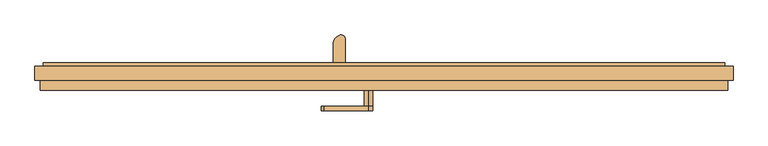
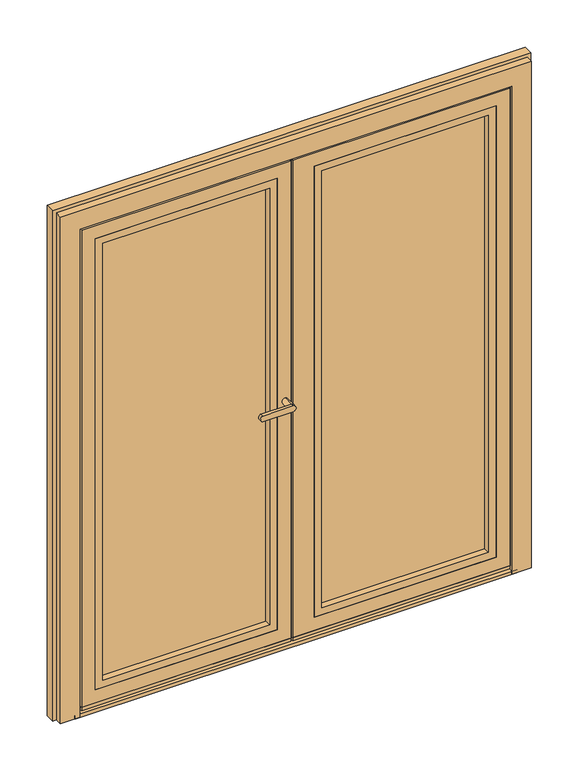
"""IFC4 building model written with IfcOpenShell, lengths in millimetres: door geometry, Schueco_FWS_ADS-75-BL-SimplySmart_out_Family-02 : FWS SI insert unit."""

from ifc_helpers import new_model, si_unit, point, frame, frame_2d, origin, place, context, project, spatial, polyline, circle_curve, ellipse_curve, trimmed, segment, composite_curve, outline, extrude, faceted_brep, source, transform, mapped, element, save
from ifc_brep_helpers import plane_surface, cylinder_surface, extruded_surface, advanced_brep


def door_16c4306f(model_context):
    return source(origin(), model_context, "Body", "SolidModel", [
        faceted_brep([(855.0, -57.5000065, 40.0), (855.0, -57.5000065, 2055.0), (855.0, -66.0002823, 2055.0), (855.0, -66.0002823, 40.0), (-12.5, -66.0002823, 40.0), (-12.5, -57.5000065, 40.0), (8.5, -57.5000065, 40.0), (865.0, -57.5000065, 30.0), (865.0, -57.5000065, 2065.0), (8.5, -57.5000065, 2065.0), (8.5, -57.5000065, 2055.0), (8.5, -57.5000065, 30.0), (-12.5, -66.0002823, 2055.0), (73.5, -66.0002823, 95.0), (73.5, -66.0002823, 2000.0), (800.0, -66.0002823, 2000.0), (800.0, -66.0002823, 95.0), (800.0, -2.0002726, 2000.0), (800.0, -2.0002726, 95.0), (73.5, -2.0002726, 95.0), (73.5, -2.0002726, 2000.0), (105.5, -2.0002726, 127.0), (105.5, -2.0002726, 1968.0), (768.0, -2.0002726, 1968.0), (768.0, -2.0002726, 127.0), (768.0, 8.9997177, 1968.0), (768.0, 8.9997177, 127.0), (105.5, 8.9997177, 127.0), (105.5, 8.9997177, 1968.0), (887.0, 8.9997177, 8.0), (19.5, 8.9997177, 8.0), (19.5, 8.9997177, 2087.0), (887.0, 8.9997177, 2087.0), (887.0, 0.4997603, 2087.0), (887.0, 0.4997603, 8.0), (19.5, 0.4997603, 8.0), (19.5, 0.4997603, 2087.0), (19.5, 0.4997603, 2065.0), (865.0, 0.4997603, 2065.0), (865.0, 0.4997603, 30.0), (19.5, 0.4997603, 30.0), (8.5, 0.4997603, 30.0), (8.5, 0.4997603, 2065.0), (-12.5, -57.5000065, 2055.0)], [[[0, 1, 2, 3]], [[3, 4, 5, 6, 0]], [[7, 8, 9, 10, 1, 0, 6, 11]], [[2, 12, 4, 3], [13, 14, 15, 16]], [[16, 15, 17, 18]], [[18, 19, 13, 16]], [[19, 20, 14, 13]], [[18, 17, 20, 19], [21, 22, 23, 24]], [[24, 23, 25, 26]], [[26, 27, 21, 24]], [[27, 28, 22, 21]], [[29, 30, 31, 32], [26, 25, 28, 27]], [[29, 32, 33, 34]], [[34, 35, 30, 29]], [[33, 36, 37, 38, 39, 40, 35, 34]], [[39, 38, 8, 7]], [[7, 11, 41, 40, 39]], [[11, 6, 10, 9, 42, 41]], [[1, 10, 43, 12, 2]], [[20, 17, 15, 14]], [[28, 25, 23, 22]], [[32, 31, 36, 33]], [[9, 8, 38, 37, 42]], [[43, 10, 6, 5]], [[4, 12, 43, 5]], [[37, 36, 31, 30, 35, 40]], [[40, 41, 42, 37]]]),
        extrude(outline(polyline([(95.0, 73.5), (95.0, 800.0), (2000.0, 800.0), (2000.0, 73.5), (95.0, 73.5)]), holes=[polyline([(125.0, 770.0), (125.0, 103.5), (1970.0, 103.5), (1970.0, 770.0), (125.0, 770.0)])]), frame((0.0, -66.0002823, 0.0), z_axis=(0.0, 1.0, 0.0), x_axis=(0.0, 0.0, 1.0)), (0.0, 0.0, 1.0), 26.0000097),
        extrude(outline(polyline([(73.5, -40.0002726), (73.5, -2.0002726), (800.0, -2.0002726), (800.0, -40.0002726), (73.5, -40.0002726)])), frame((0.0, 0.0, 95.0), z_axis=(0.0, 0.0, 1.0), x_axis=(1.0, 0.0, 0.0)), (0.0, 0.0, 1.0), 1905.0),
        extrude(outline(polyline([(855.0, -66.0002823), (-12.5, -66.0002823), (-12.5, -57.5003249), (855.0, -57.5003249), (855.0, -66.0002823)])), frame((0.0, 0.0, 26.0), z_axis=(0.0, 0.0, 1.0), x_axis=(1.0, 0.0, 0.0)), (0.0, 0.0, 1.0), 14.0),
        extrude(outline(composite_curve([segment(polyline([(-139.1673236, 8.9997177), (-139.1673236, 59.1618682)]), True, "CONTINUOUS"), segment(trimmed(circle_curve(frame_2d((-111.9889059, 59.1618682)), 27.1784177), [point((-139.1673236, 59.1618682))], [point((-121.5260015, 84.6120194))], False, "CARTESIAN"), True, "CONTINUOUS"), segment(trimmed(circle_curve(frame_2d((-117.4485005, 73.7310321)), 11.6198924), [point((-121.5260015, 84.6120194))], [point((-105.8286081, 73.7310321))], False, "CARTESIAN"), True, "CONTINUOUS"), segment(polyline([(-105.8286081, 73.7310321), (-105.8286081, 8.9997177), (-139.1673236, 8.9997177)]), True, "CONTINUOUS")], self_intersect=False)), frame((0.0, 0.0, 2030.9340013), z_axis=(0.0, 0.0, 1.0), x_axis=(1.0, 0.0, 0.0)), (0.0, 0.0, 1.0), 4.0),
        extrude(outline(polyline([(-139.1673236, 12.9997177), (-105.8286081, 12.9997177), (-105.8286081, 8.9997177), (-139.1673236, 8.9997177), (-139.1673236, 12.9997177)])), frame((0.0, 0.0, 2000.9340013), z_axis=(0.0, 0.0, 1.0), x_axis=(1.0, 0.0, 0.0)), (0.0, 0.0, 1.0), 30.0),
        extrude(outline(polyline([(-139.1673236, 12.9997177), (-105.8286081, 12.9997177), (-105.8286081, 8.9997177), (-139.1673236, 8.9997177), (-139.1673236, 12.9997177)])), frame((0.0, 0.0, 56.9340013), z_axis=(0.0, 0.0, 1.0), x_axis=(1.0, 0.0, 0.0)), (0.0, 0.0, 1.0), 30.0),
        extrude(outline(composite_curve([segment(polyline([(-139.1673236, 8.9997177), (-139.1673236, 59.1618682)]), True, "CONTINUOUS"), segment(trimmed(circle_curve(frame_2d((-111.9889059, 59.1618682)), 27.1784177), [point((-139.1673236, 59.1618682))], [point((-121.5260015, 84.6120194))], False, "CARTESIAN"), True, "CONTINUOUS"), segment(trimmed(circle_curve(frame_2d((-117.4485005, 73.7310321)), 11.6198924), [point((-121.5260015, 84.6120194))], [point((-105.8286081, 73.7310321))], False, "CARTESIAN"), True, "CONTINUOUS"), segment(polyline([(-105.8286081, 73.7310321), (-105.8286081, 8.9997177), (-139.1673236, 8.9997177)]), True, "CONTINUOUS")], self_intersect=False)), frame((0.0, 0.0, 52.9340013), z_axis=(0.0, 0.0, 1.0), x_axis=(1.0, 0.0, 0.0)), (0.0, 0.0, 1.0), 4.0),
        advanced_brep(
        [(-109.782924, 57.5977179, 2030.9340013), (-135.217076, 72.2821425, 2030.9340013), (-109.782924, 57.5977179, 56.9340013), (-135.217076, 72.2821425, 56.9340013)],
        [
            (0, 1, ellipse_curve(frame((-122.5, 64.9399302, 2030.9340013), z_axis=(0.0, 0.0, 1.0000000000000002), x_axis=(0.5000002582658958, 0.866025254674503, 0.0)), 21.5840887, 14.6844171)),
            (1, 0, ellipse_curve(frame((-122.5, 64.9399302, 2030.9340013), z_axis=(0.0, 0.0, 1.0000000000000002), x_axis=(0.5000002582658958, 0.866025254674503, 0.0)), 21.5840887, 14.6844171)),
            (2, 3, ellipse_curve(frame((-122.5, 64.9399302, 56.9340013), z_axis=(0.0, 0.0, -1.0000000000000002), x_axis=(-0.866025254674503, 0.5000002582658958, 0.0)), 14.6844171, 21.5840887)),
            (3, 2, ellipse_curve(frame((-122.5, 64.9399302, 56.9340013), z_axis=(0.0, 0.0, -1.0000000000000002), x_axis=(-0.866025254674503, 0.5000002582658958, 0.0)), 14.6844171, 21.5840887)),
            (0, 2),
            (3, 1),
        ],
        [
            plane_surface(frame((-135.217076, 72.2821425, 2030.9340013), z_axis=(0.0, 0.0, 1.0000000000000002), x_axis=(0.5000002582658958, 0.866025254674503, 0.0))),
            plane_surface(frame((-135.217076, 72.2821425, 56.9340013), z_axis=(0.0, 0.0, -1.0000000000000002), x_axis=(-0.5000002582658958, -0.866025254674503, 0.0))),
            extruded_surface(trimmed(ellipse_curve(frame((-122.5, 64.9399302, 56.9340013), z_axis=(0.0, 0.0, -1.0000000000000002), x_axis=(-0.866025254674503, 0.5000002582658958, 0.0)), 14.6844171, 21.5840887), [point((-135.217076, 72.2821425, 56.9340013))], [point((-109.782924, 57.5977179, 56.9340013))], True, "CARTESIAN"), (0.0, 0.0, -1974.0), 1974.0),
            extruded_surface(trimmed(ellipse_curve(frame((-122.5, 64.9399302, 56.9340013), z_axis=(0.0, 0.0, -1.0000000000000002), x_axis=(-0.866025254674503, 0.5000002582658958, 0.0)), 14.6844171, 21.5840887), [point((-109.782924, 57.5977179, 56.9340013))], [point((-135.217076, 72.2821425, 56.9340013))], True, "CARTESIAN"), (0.0, 0.0, -1974.0), 1974.0),
        ],
        [
            (0, [[1, 2]]),
            (1, [[3, 4]]),
            (2, [[5, -4, 6, -1]]),
            (3, [[-6, -3, -5, -2]]),
        ],
    ),
        advanced_brep(
        [(-42.5, -122.0002518, 1038.0113692), (-42.5, -122.0002518, 1061.9886308), (-164.1617926, -122.0002518, 1061.9886308), (-164.1617926, -122.0002518, 1038.0113692), (-42.5, -109.5001648, 1061.9886308), (-42.5, -109.5001648, 1038.0113692), (-164.1617926, -109.5001648, 1038.0113692), (-164.1617926, -109.5001648, 1061.9886308), (-42.5, -66.0002823, 1038.0113692), (-42.5, -66.0002823, 1061.9886308)],
        [
            (0, 1, circle_curve(frame((-42.5, -122.0002518, 1050.0), z_axis=(0.0, -1.0, 0.0), x_axis=(0.0, 0.0, 1.0)), 11.9886308)),
            (1, 2),
            (2, 3, ellipse_curve(frame((-164.1617926, -122.0002518, 1050.0), z_axis=(0.0, -1.0, 0.0), x_axis=(0.0, 0.0, -1.0)), 11.9886308, 7.9050795)),
            (3, 0),
            (4, 5, circle_curve(frame((-42.5, -109.5001648, 1050.0), z_axis=(0.0, -1.0, 0.0), x_axis=(0.0, 0.0, 1.0)), 11.9886308)),
            (5, 6),
            (6, 7, ellipse_curve(frame((-164.1617926, -109.5001648, 1050.0), z_axis=(0.0, 1.0, 0.0), x_axis=(0.0, 0.0, -1.0)), 11.9886308, 7.9050795)),
            (7, 4),
            (3, 6),
            (5, 0),
            (2, 7),
            (1, 4),
            (5, 4, circle_curve(frame((-42.5, -109.5001648, 1050.0), z_axis=(0.0, -1.0, 0.0), x_axis=(0.0, 0.0, 1.0)), 11.9886308)),
            (8, 9, circle_curve(frame((-42.5, -66.0002823, 1050.0), z_axis=(0.0, 1.0, 0.0), x_axis=(0.0, 0.0, 1.0)), 11.9886308)),
            (9, 8, circle_curve(frame((-42.5, -66.0002823, 1050.0), z_axis=(0.0, 1.0, 0.0), x_axis=(0.0, 0.0, 1.0)), 11.9886308)),
            (8, 5),
            (4, 9),
        ],
        [
            plane_surface(frame((-164.1617926, -122.0002518, 1038.0113692), z_axis=(0.0, -1.0, 0.0), x_axis=(-1.0, 0.0, 0.0))),
            plane_surface(frame((-164.1617926, -109.5001648, 1038.0113692), z_axis=(0.0, 1.0, 0.0), x_axis=(1.0, 0.0, 0.0))),
            plane_surface(frame((-42.5, -122.0002518, 1038.0113692), z_axis=(0.0, 0.0, -1.0), x_axis=(0.0, 1.0, 0.0))),
            extruded_surface(trimmed(ellipse_curve(frame((-164.1617926, -109.5001648, 1050.0), z_axis=(0.0, 1.0, 0.0), x_axis=(0.0, 0.0, -1.0)), 11.9886308, 7.9050795), [point((-164.1617926, -109.5001648, 1038.0113692))], [point((-164.1617926, -109.5001648, 1061.9886308))], True, "CARTESIAN"), (0.0, 12.500086999999994, 0.0), 12.500086999999994),
            plane_surface(frame((-164.1617926, -122.0002518, 1061.9886308), z_axis=(0.0, 0.0, 1.0), x_axis=(0.0, 1.0, 0.0))),
            cylinder_surface(frame((-42.5, -109.5001648, 1050.0), z_axis=(0.0, -1.0, 0.0), x_axis=(0.0, 0.0, 1.0)), 11.9886308),
            plane_surface(frame((-42.5, -66.0002823, 1061.9886308), z_axis=(0.0, 1.0, 0.0), x_axis=(-1.0, 0.0, 0.0))),
            cylinder_surface(frame((-42.5, -66.0002823, 1050.0), z_axis=(0.0, -1.0, 0.0), x_axis=(0.0, 0.0, 1.0)), 11.9886308),
        ],
        [
            (0, [[1, 2, 3, 4]]),
            (1, [[5, 6, 7, 8]]),
            (2, [[9, -6, 10, -4]]),
            (3, [[11, -7, -9, -3]]),
            (4, [[12, -8, -11, -2]]),
            (5, [[-10, 13, -12, -1]]),
            (6, [[14, 15]]),
            (7, [[16, -5, 17, -14]]),
            (7, [[-17, -13, -16, -15]]),
        ],
    ),
        faceted_brep([(-855.0, -57.5000065, 40.0), (-855.0, -66.0002823, 40.0), (-855.0, -66.0002823, 2055.0), (-855.0, -57.5000065, 2055.0), (-29.5, -57.5000065, 40.0), (-19.5, -57.5000065, 40.0), (-19.5, -66.0002823, 40.0), (-29.5, -66.0002823, 40.0), (-865.0, -57.5000065, 30.0), (-9.5, -57.5000065, 30.0), (-9.5, -57.5000065, 2065.0), (-865.0, -57.5000065, 2065.0), (-19.5, -57.5000065, 2055.0), (-29.5, -57.5000065, 2055.0), (-19.5, -66.0002823, 2055.0), (-29.5, -66.0002823, 2055.0), (-74.5, -66.0002823, 95.0), (-800.0, -66.0002823, 95.0), (-800.0, -66.0002823, 2000.0), (-74.5, -66.0002823, 2000.0), (-800.0, -2.0002726, 95.0), (-800.0, -2.0002726, 2000.0), (-74.5, -2.0002726, 95.0), (-74.5, -2.0002726, 2000.0), (-106.5, -2.0002726, 127.0), (-768.0, -2.0002726, 127.0), (-768.0, -2.0002726, 1968.0), (-106.5, -2.0002726, 1968.0), (-768.0, 8.9997177, 127.0), (-768.0, 8.9997177, 1968.0), (-106.5, 8.9997177, 127.0), (-106.5, 8.9997177, 1968.0), (12.5, 8.9997177, 8.0), (-887.0, 8.9997177, 8.0), (-887.0, 8.9997177, 2087.0), (12.5, 8.9997177, 2087.0), (-887.0, 0.4997603, 8.0), (-887.0, 0.4997603, 2087.0), (12.5, 0.4997603, 8.0), (12.5, 0.4997603, 2087.0), (-9.5, 0.4997603, 30.0), (-865.0, 0.4997603, 30.0), (-865.0, 0.4997603, 2065.0), (-9.5, 0.4997603, 2065.0)], [[[0, 1, 2, 3]], [[1, 0, 4, 5, 6, 7]], [[8, 9, 10, 11], [12, 5, 4, 0, 3, 13]], [[6, 5, 12, 14]], [[6, 14, 15, 2, 1, 7], [16, 17, 18, 19]], [[17, 20, 21, 18]], [[20, 17, 16, 22]], [[22, 16, 19, 23]], [[20, 22, 23, 21], [24, 25, 26, 27]], [[25, 28, 29, 26]], [[28, 25, 24, 30]], [[30, 24, 27, 31]], [[32, 33, 34, 35], [28, 30, 31, 29]], [[33, 36, 37, 34]], [[36, 33, 32, 38]], [[38, 32, 35, 39]], [[36, 38, 39, 37], [40, 41, 42, 43]], [[41, 8, 11, 42]], [[8, 41, 40, 9]], [[9, 40, 43, 10]], [[14, 12, 13, 3, 2, 15]], [[23, 19, 18, 21]], [[31, 27, 26, 29]], [[39, 35, 34, 37]], [[10, 43, 42, 11]]]),
        extrude(outline(polyline([(95.0, -74.5), (2000.0, -74.5), (2000.0, -800.0), (95.0, -800.0), (95.0, -74.5)]), holes=[polyline([(125.0, -770.0), (1970.0, -770.0), (1970.0, -104.5), (125.0, -104.5), (125.0, -770.0)])]), frame((0.0, -66.0002823, 0.0), z_axis=(0.0, 1.0, 0.0), x_axis=(0.0, 0.0, 1.0)), (0.0, 0.0, 1.0), 26.0000097),
        extrude(outline(polyline([(-74.5, -40.0002726), (-800.0, -40.0002726), (-800.0, -2.0002726), (-74.5, -2.0002726), (-74.5, -40.0002726)])), frame((0.0, 0.0, 95.0), z_axis=(0.0, 0.0, 1.0), x_axis=(1.0, 0.0, 0.0)), (0.0, 0.0, 1.0), 1905.0),
        extrude(outline(polyline([(-855.0, -66.0002823), (-855.0, -57.5003249), (-19.5, -57.5003249), (-19.5, -66.0002823), (-855.0, -66.0002823)])), frame((0.0, 0.0, 26.0), z_axis=(0.0, 0.0, 1.0), x_axis=(1.0, 0.0, 0.0)), (0.0, 0.0, 1.0), 14.0),
        faceted_brep([(930.999943, 8.9997177, 2130.999943), (930.999943, 0.0, 2130.999943), (930.999943, 0.0, 0.0), (930.999943, 8.9997177, 0.0), (-954.0, 0.0, 0.0), (-954.0, 0.0, 2154.0), (954.0, 0.0, 2154.0), (954.0, 0.0, 0.0), (-930.999943, 0.0, 2130.999943), (-930.999943, 0.0, 0.0), (954.0, -38.0, 0.0), (940.0, -38.0, 0.0), (940.0, -66.0002823, 0.0), (861.9999732, -66.0002823, 0.0), (861.9999732, -57.5000065, 0.0), (882.4999732, -57.5000065, 0.0), (882.4999732, 0.4997603, 0.0), (893.9999732, 0.4997603, 0.0), (893.9999732, 8.9997177, 0.0), (-893.9999732, 8.9997177, 0.0), (-930.999943, 8.9997177, 0.0), (-930.999943, 8.9997177, 2130.999943), (893.9999732, 8.9997177, 2093.9999732), (-893.9999732, 8.9997177, 2093.9999732), (861.9999732, -66.0002823, 2061.9999732), (861.9999732, -57.5000065, 2061.9999732), (-861.9999732, -57.5000065, 0.0), (-882.4999732, -57.5000065, 0.0), (-882.4999732, -57.5000065, 2082.4999732), (882.4999732, -57.5000065, 2082.4999732), (-861.9999732, -57.5000065, 2061.9999732), (-940.0, -66.0002823, 0.0), (-861.9999732, -66.0002823, 0.0), (-861.9999732, -66.0002823, 2061.9999732), (940.0, -66.0002823, 2140.0), (-940.0, -66.0002823, 2140.0), (940.0, -38.0, 2140.0), (-954.0, -38.0, 0.0), (-940.0, -38.0, 0.0), (-940.0, -38.0, 2140.0), (954.0, -38.0, 2154.0), (-954.0, -38.0, 2154.0), (-893.9999732, 0.4997603, 0.0), (-882.4999732, 0.4997603, 0.0), (893.9999732, 0.4997603, 2093.9999732), (-893.9999732, 0.4997603, 2093.9999732), (882.4999732, 0.4997603, 2082.4999732), (-882.4999732, 0.4997603, 2082.4999732)], [[[0, 1, 2, 3]], [[4, 5, 6, 7, 2, 1, 8, 9]], [[3, 2, 7, 10, 11, 12, 13, 14, 15, 16, 17, 18]], [[19, 20, 21, 0, 3, 18, 22, 23]], [[24, 25, 14, 13]], [[26, 27, 28, 29, 15, 14, 25, 30]], [[31, 32, 33, 24, 13, 12, 34, 35]], [[34, 12, 11, 36]], [[37, 38, 39, 36, 11, 10, 40, 41]], [[4, 9, 20, 19, 42, 43, 27, 26, 32, 31, 38, 37]], [[20, 9, 8, 21]], [[18, 17, 44, 22]], [[42, 19, 23, 45]], [[32, 26, 30, 33]], [[31, 35, 39, 38]], [[4, 37, 41, 5]], [[6, 40, 10, 7]], [[43, 42, 45, 44, 17, 16, 46, 47]], [[16, 15, 29, 46]], [[27, 43, 47, 28]], [[21, 8, 1, 0]], [[33, 30, 25, 24]], [[35, 34, 36, 39]], [[23, 22, 44, 45]], [[5, 41, 40, 6]], [[47, 46, 29, 28]]]),
        extrude(outline(polyline([(0.4997603, 16.5), (0.4997603, 0.0), (-66.0002823, 0.0), (-66.0002823, 13.2855157), (-46.5000038, 20.0), (-44.0000038, 20.0), (-44.0000038, 16.5), (0.4997603, 16.5)])), frame((-882.4999732, 0.0, 0.0), z_axis=(1.0, 0.0, 0.0), x_axis=(0.0, 1.0, 0.0)), (0.0, 0.0, 1.0), 1764.9999465),
    ])


if __name__ == "__main__":
    model = new_model("IFC4")
    model_context = context("Model", 3, world=origin())
    ifc_project = project(units=[si_unit("LENGTHUNIT", "METRE", prefix="MILLI")], contexts=[model_context])
    site = spatial("IfcSite", under=ifc_project)
    building = spatial("IfcBuilding", under=site)
    placement = place(None, origin())
    door_shape = door_16c4306f(model_context)
    element("IfcDoor", 1, ObjectType="Schueco_FWS_ADS-75-BL-SimplySmart_out_Family-02 : FWS SI insert unit", at=placement, inside=building, context=model_context, shape_type="MappedRepresentation", body=[
        mapped(door_shape, transform((0.0, 0.0, 0.0), x_axis=(1.0, 0.0, 0.0), y_axis=(0.0, 1.0, 0.0), z_axis=(0.0, 0.0, 1.0))),
    ])
    save(model, "model.ifc")

# Revit data of these elements
# Type "Schueco_FWS_ADS-75-BL-SimplySmart_out_Family-02 : FWS SI insert unit"
#   Type Mark = "33"
#   __NOTE__ = "Data describes the optimum values of the entire system. The properites of a selected design option have to be determined on an individual basis!"
#   Wind load resistance = "Class C3"
#   Watertightness = "Class E750"
#   Thermal insulation = "Uf = 1.6 W/(m²K)"
#   Sound insulation = "..."
#   Schueco thermal insulation standard = "Highly thermally insulated"
#   Opening type = "Outward-opening, Flush-fitted"
#   Model = "Schueco ADS 75 BL SimplySmart"
#   Mechanical loading = "..."
#   Maximum leaf width in mm = "1400"
#   Maximum leaf weight in kg = "200"
#   Maximum leaf height in mm = "3000"
#   Material = "Aluminium"
#   Construction Type = "Door, double-leaf, outward-opening"
#   Manufacturer = "Schueco International KG"
#   Long term functionality = "..."
#   Glazing data = "Triple glazing 38mm"
#   Façade insert unit = "yes"
#   Family creation date = "08.2017"
#   Description = "Schueco Aluminium Door System (ADS)"
#   Burglar resistance = "Class RC 2"
#   Areas of use = "Public buildings, Residential buildings, Side entrance"
#   Analytic Construction = "<None>"
#   Air permeability = "Class 4"
#   Width [instance default] = 981.242 mm
#   Leaf opening angle [instance default] = 0.00°
#   IOf_T = 38 mm
#   Height [instance default] = 1923.399 mm
#   Glazing area [instance default] = 0.639718 m²
#   F2_W [instance default] = 491.621 mm
#   F1_W [instance default] = 490.621 mm
#   Distance from bottom to handles [instance default] = 1050 mm
#   Clear opening width [instance default] = 797.242 mm
#   Active leaf width = 1100 mm
#   Standard threshold = yes
#   Low level threshold = no
#   Handles = yes
#   FWS SI insert unit = yes
#   FWS HI insert unit = no
#   All fields of identical width = yes
#   Glass = none
#   Frame = Alu
#   Fittings = none
# Element 1 (IfcDoor, "Schueco_FWS_ADS-75-BL-SimplySmart_out_Family-02 : FWS SI insert unit")
#   Width = 1908 mm
#   Height = 2154 mm
#   Glazing area = 2.43748 m²
#   F2_W = 955 mm
#   F1_W = 954 mm
#   Clear opening width = 1724 mm
#   Materials on its faces: "Alu", "Glass"
# Materials
#   "Alu": class "Glas", colour RGB 140 140 140, transparency 0
#   "Glass": class "Glass", colour RGB 128 128 255, transparency 0.75, Description = "Soda Lime Glass", Cost = 0
